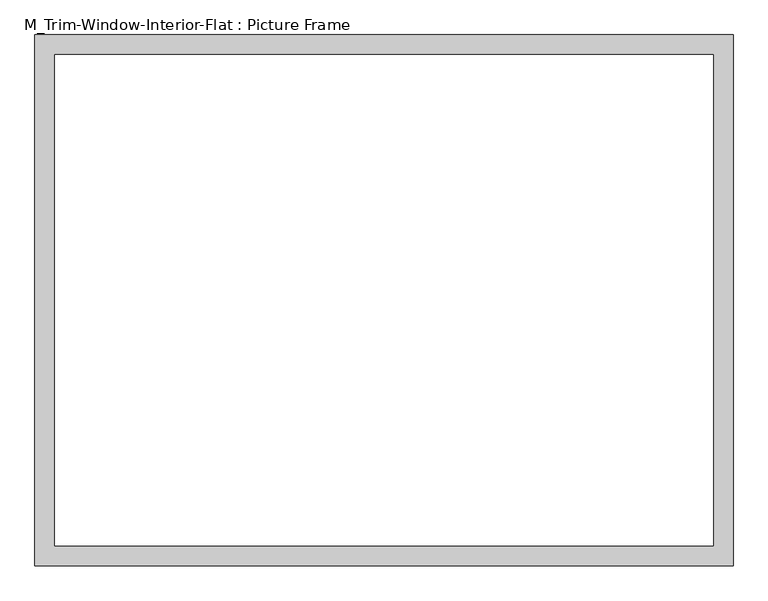
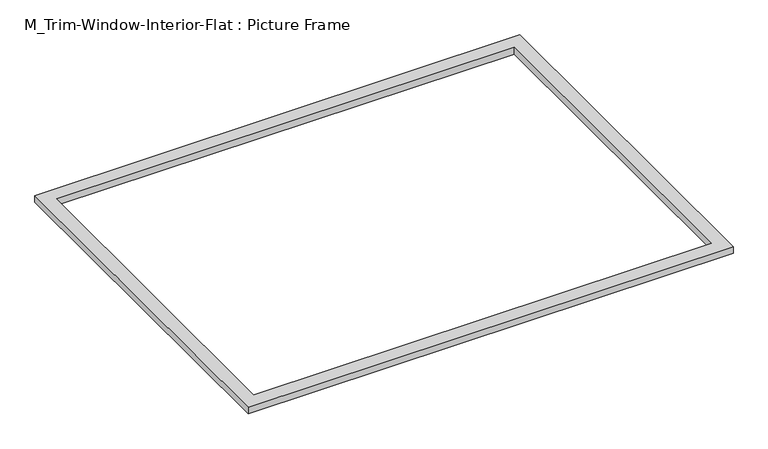
"""IFC4 building model written with IfcOpenShell, lengths in millimetres: proxy geometry, M_Trim-Window-Interior-Flat : Picture Frame."""

from ifc_helpers import new_model, si_unit, origin, origin_with_axes, place, context, project, spatial, polyline, outline, extrude, source, transform, mapped, element, save


def m_trim_window_interior_flat_picture_frame_ad33684f(model_context):
    return source(origin(), model_context, "Body", "SweptSolid", [
        extrude(outline(polyline([(1047.3, 47.3), (1047.3, -1547.3), (-1047.3, -1547.3), (-1047.3, 47.3), (1047.3, 47.3)]), holes=[polyline([(987.3, -12.7), (-987.3, -12.7), (-987.3, -1487.3), (987.3, -1487.3), (987.3, -12.7)])]), origin_with_axes(), (0.0, 0.0, 1.0), 30.0),
    ])


if __name__ == "__main__":
    model = new_model("IFC4")
    model_context = context("Model", 3, world=origin())
    ifc_project = project(units=[si_unit("LENGTHUNIT", "METRE", prefix="MILLI")], contexts=[model_context])
    site = spatial("IfcSite", under=ifc_project)
    building = spatial("IfcBuilding", under=site)
    placement = place(None, origin())
    m_trim_window_interior_flat_picture_frame_shape = m_trim_window_interior_flat_picture_frame_ad33684f(model_context)
    element("IfcBuildingElementProxy", 1, Name="M_Trim-Window-Interior-Flat : Picture Frame", ObjectType="M_Trim-Window-Interior-Flat : Picture Frame", at=placement, inside=building, context=model_context, shape_type="MappedRepresentation", body=[
        mapped(m_trim_window_interior_flat_picture_frame_shape, transform((0.0, 0.0, 0.0), x_axis=(1.0, 0.0, 0.0), y_axis=(0.0, 1.0, 0.0), z_axis=(0.0, 0.0, 1.0))),
    ])
    save(model, "model.ifc")

# Revit data of these elements
# Type "M_Trim-Window-Interior-Flat : Picture Frame"
#   Trim Thickness_Picture Frame = 30 mm
#   Trim Width = 60 mm
#   Trim Thickness_with Sill = 20 mm
#   Sill Thickness = 30 mm
#   Opening Width [instance default] = 600 mm
#   Opening Height [instance default] = 900 mm
#   Default Elevation = 1200 mm
#   Sill = no
#   Picture Frame = yes
#   Trim Material [instance default] = none
# Element 1 (IfcBuildingElementProxy, "M_Trim-Window-Interior-Flat : Picture Frame")
#   Opening Width = 2000 mm
#   Opening Height = 1500 mm
#   Trim Material = Wood - Stained
#   Materials on its faces: "Wood - Stained"
# Materials
#   "Wood - Stained": class "Wood", colour RGB 173 132 96, transparency 0, Cost = 0
